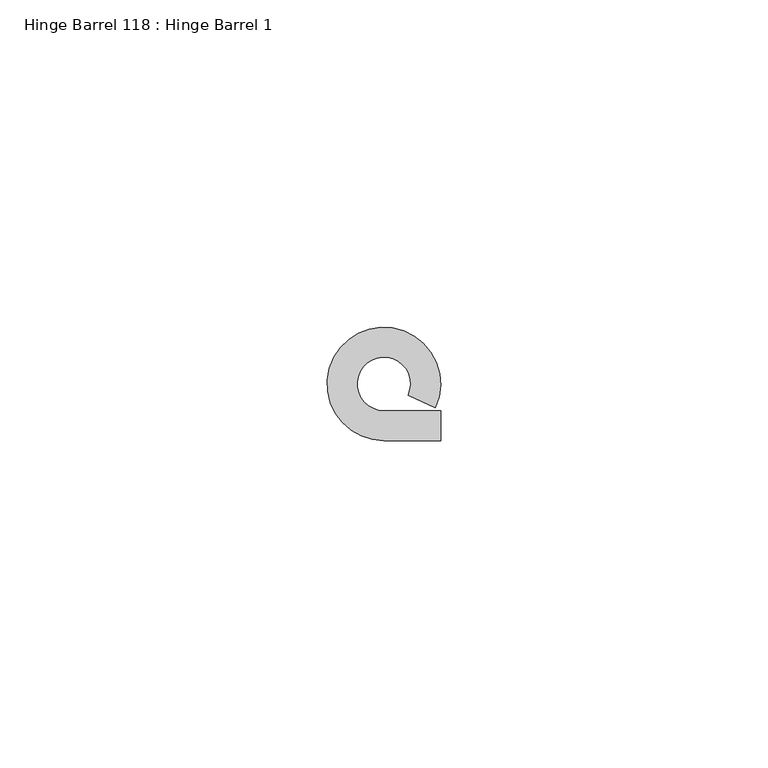
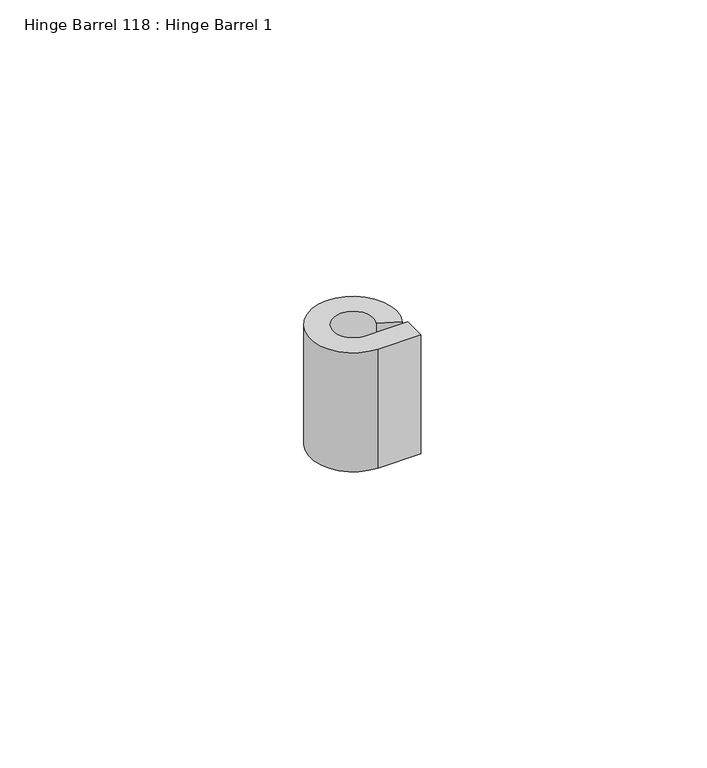
"""IFC4 building model written with IfcOpenShell, lengths in millimetres: proxy geometry, Hinge Barrel 118 : Hinge Barrel 1."""

from ifc_helpers import new_model, si_unit, point, frame, frame_2d, origin, place, context, project, spatial, polyline, circle_curve, trimmed, segment, composite_curve, outline, extrude, source, transform, mapped, element, save


def hinge_barrel_118_hinge_barrel_1_0a67a66c(model_context):
    return source(origin(), model_context, "Body", "SweptSolid", [
        extrude(outline(composite_curve([segment(polyline([(587323.2214739, -534104.7943841), (587327.7934739, -534104.7943841), (587327.7934739, -534109.3584466), (587319.1320739, -534109.3584466)]), True, "CONTINUOUS"), segment(trimmed(circle_curve(frame_2d((587319.1320739, -534100.7049841)), 8.6534625), [point((587319.1320739, -534109.3584466))], [point((587326.986084, -534104.3377433))], False, "CARTESIAN"), True, "CONTINUOUS"), segment(polyline([(587326.986084, -534104.3377433), (587322.8436736, -534102.421731)]), True, "CONTINUOUS"), segment(trimmed(circle_curve(frame_2d((587319.1320739, -534100.7049841)), 4.0894), [point((587322.8436736, -534102.421731))], [point((587319.1320739, -534104.7943841))], True, "CARTESIAN"), True, "CONTINUOUS"), segment(polyline([(587319.1320739, -534104.7943841), (587323.2214739, -534104.7943841)]), True, "CONTINUOUS")], self_intersect=False)), frame((0.0, 0.0, 2038.35), z_axis=(0.0, 0.0, 1.0), x_axis=(1.0, 0.0, 0.0)), (0.0, 0.0, 1.0), 25.4),
    ])


if __name__ == "__main__":
    model = new_model("IFC4")
    model_context = context("Model", 3, world=origin())
    ifc_project = project(units=[si_unit("LENGTHUNIT", "METRE", prefix="MILLI")], contexts=[model_context])
    site = spatial("IfcSite", under=ifc_project)
    building = spatial("IfcBuilding", under=site)
    placement = place(None, origin())
    hinge_barrel_118_hinge_barrel_1_shape = hinge_barrel_118_hinge_barrel_1_0a67a66c(model_context)
    element("IfcBuildingElementProxy", 1, Name="Hinge Barrel 118 : Hinge Barrel 1", ObjectType="Hinge Barrel 118 : Hinge Barrel 1", at=placement, inside=building, context=model_context, shape_type="MappedRepresentation", body=[
        mapped(hinge_barrel_118_hinge_barrel_1_shape, transform((0.0, 0.0, 0.0), x_axis=(1.0, 0.0, 0.0), y_axis=(0.0, 1.0, 0.0), z_axis=(0.0, 0.0, 1.0))),
    ])
    save(model, "model.ifc")

# Revit data of these elements
# Element 1 (IfcBuildingElementProxy, "Hinge Barrel 118 : Hinge Barrel 1")
#   Materials on its faces: "6\"X6\" WELD-ON STL BUTT HINGE"
# Materials
#   "6\"X6\" WELD-ON STL BUTT HINGE": class "Metal", colour RGB 189 187 185, transparency 0, Description = "Carbon steel", Cost = 0
